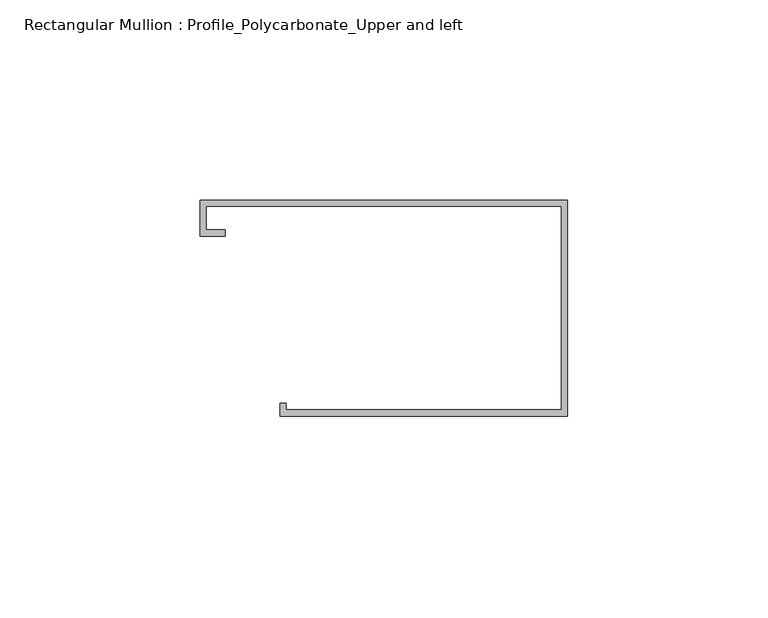
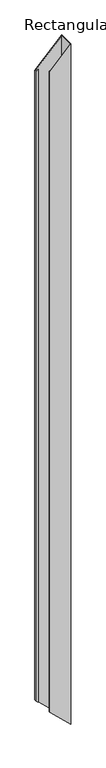
"""IFC4 building model written with IfcOpenShell, lengths in millimetres: member geometry, Rectangular Mullion : Profile_Polycarbonate_Upper and left."""

from ifc_helpers import new_model, si_unit, origin, place, context, project, spatial, faceted_brep, source, transform, mapped, element, save


def rectangular_mullion_profile_polycarbonate_upper_and_left_07825f8f(model_context):
    return source(origin(), model_context, "Body", "Brep", [
        faceted_brep([(-91.9988, 28.984575, -95.9119088), (0.0, 28.984575, 0.0), (0.0, 28.984575, -2459.5822781), (-91.9988, 28.984575, -2371.336936), (-91.9988, 19.992975, -95.9119088), (-91.9988, 19.992975, -2371.336936), (-85.6488, 19.992975, -89.2918157), (-85.6488, 19.992975, -2377.4278624), (-85.6488, 21.580475, -89.2918157), (-85.6488, 21.580475, -2377.4278624), (-90.4113, 21.580475, -94.2568855), (-90.4113, 21.580475, -2372.8596676), (-90.4113, 27.397075, -94.2568855), (-90.4113, 27.397075, -2372.8596676), (-1.5875, 27.397075, -1.6550233), (-1.5875, 27.397075, -2458.0595465), (-1.5875, -23.428325, -1.6550233), (-1.5875, -23.428325, -2458.0595465), (-70.3961, -23.428325, -73.3903521), (-70.3961, -23.428325, -2392.0582677), (-70.3961, -21.840825, -73.3903521), (-70.3961, -21.840825, -2392.0582677), (-71.9836, -21.840825, -75.0453753), (-71.9836, -21.840825, -2390.5355361), (-71.9836, -25.015825, -75.0453753), (-71.9836, -25.015825, -2390.5355361), (0.0, -25.015825, 0.0), (0.0, -25.015825, -2459.5822781)], [[[0, 1, 2, 3]], [[4, 0, 3, 5]], [[6, 4, 5, 7]], [[8, 6, 7, 9]], [[10, 8, 9, 11]], [[12, 10, 11, 13]], [[14, 12, 13, 15]], [[16, 14, 15, 17]], [[18, 16, 17, 19]], [[20, 18, 19, 21]], [[22, 20, 21, 23]], [[24, 22, 23, 25]], [[26, 24, 25, 27]], [[1, 26, 27, 2]], [[1, 0, 4, 6, 8, 10, 12, 14, 16, 18, 20, 22, 24, 26]], [[2, 27, 25, 23, 21, 19, 17, 15, 13, 11, 9, 7, 5, 3]]]),
    ])


if __name__ == "__main__":
    model = new_model("IFC4")
    model_context = context("Model", 3, world=origin())
    ifc_project = project(units=[si_unit("LENGTHUNIT", "METRE", prefix="MILLI")], contexts=[model_context])
    site = spatial("IfcSite", under=ifc_project)
    building = spatial("IfcBuilding", under=site)
    placement = place(None, origin())
    rectangular_mullion_profile_polycarbonate_upper_and_left_shape = rectangular_mullion_profile_polycarbonate_upper_and_left_07825f8f(model_context)
    element("IfcMember", 1, ObjectType="Rectangular Mullion : Profile_Polycarbonate_Upper and left", at=placement, inside=building, context=model_context, shape_type="MappedRepresentation", body=[
        mapped(rectangular_mullion_profile_polycarbonate_upper_and_left_shape, transform((0.0, 0.0, 0.0), x_axis=(1.0, 0.0, 0.0), y_axis=(0.0, 1.0, 0.0), z_axis=(0.0, 0.0, 1.0))),
    ])
    save(model, "model.ifc")

# Revit data of these elements
# Type "Rectangular Mullion : Profile_Polycarbonate_Upper and left"
#   built-in parameter 1007322 = 0.177167 (stored number, unit not read)
#   built-in parameter 1007321 = 0.00520833 (stored number, unit not read)
#   built-in parameter 1007320 = 0 (stored number, unit not read)
